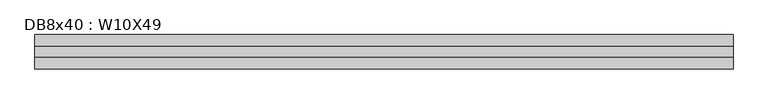
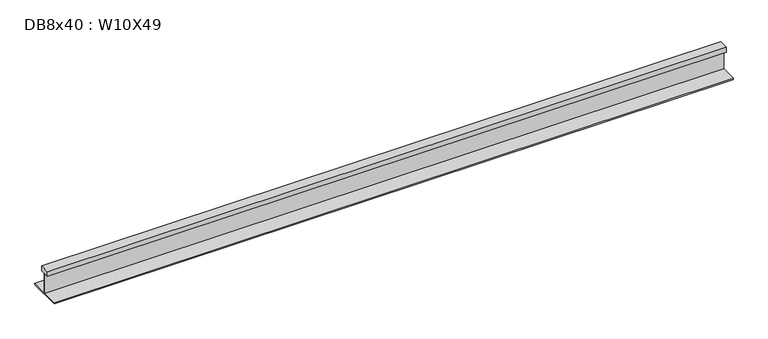
"""IFC4 building model written with IfcOpenShell, lengths in millimetres: beam geometry, DB8x40 : W10X49."""

from ifc_helpers import new_model, si_unit, frame, origin, place, context, project, spatial, polyline, outline, extrude, source, transform, mapped, element, save


def db8x40_w10x49_3a02a75a(model_context):
    return source(origin(), model_context, "Body", "SweptSolid", [
        extrude(outline(polyline([(38.1, 144.3355), (38.1, 106.2355), (2.921, 106.2355), (2.921, -49.53), (127.0, -49.53), (127.0, -59.182), (-127.0, -59.182), (-127.0, -49.53), (-2.921, -49.53), (-2.921, 106.2355), (-38.1, 106.2355), (-38.1, 144.3355), (38.1, 144.3355)])), frame((-2504.8176847, 0.0, 0.0), z_axis=(1.0, 0.0, 0.0), x_axis=(0.0, 1.0, 0.0)), (0.0, 0.0, 1.0), 5146.3938722),
    ])


if __name__ == "__main__":
    model = new_model("IFC4")
    model_context = context("Model", 3, world=origin())
    ifc_project = project(units=[si_unit("LENGTHUNIT", "METRE", prefix="MILLI")], contexts=[model_context])
    site = spatial("IfcSite", under=ifc_project)
    building = spatial("IfcBuilding", under=site)
    placement = place(None, origin())
    db8x40_w10x49_shape = db8x40_w10x49_3a02a75a(model_context)
    element("IfcBeam", 1, ObjectType="DB8x40 : W10X49", at=placement, inside=building, context=model_context, shape_type="MappedRepresentation", body=[
        mapped(db8x40_w10x49_shape, transform((0.0, 0.0, 0.0), x_axis=(1.0, 0.0, 0.0), y_axis=(0.0, 1.0, 0.0), z_axis=(0.0, 0.0, 1.0))),
    ])
    save(model, "model.ifc")

# Revit data of these elements
# Type "DB8x40 : W10X49"
#   Assembly Code = "B10"
#   W = 53
#   Length [instance default] = 5' - 0"
#   bf = 0' - 10"
#   d = 1' - 0.1"
#   k = 0' - 1 3/8"
#   k2 = 0' - 0.8"
#   tf = 0' - 0.575"
#   tw = 0' - 0.345"
#   A = 0.108333 SF
#   Structural Material [instance default] = Steel ASTM A992
# Element 1 (IfcBeam, "DB8x40 : W10X49")
#   Materials on its faces: "Steel ASTM A992"
# Materials
#   "Steel ASTM A992": class "Metal", colour RGB 199 199 199, transparency 0, Description = "Structural steel 50ksi", Cost = 0
